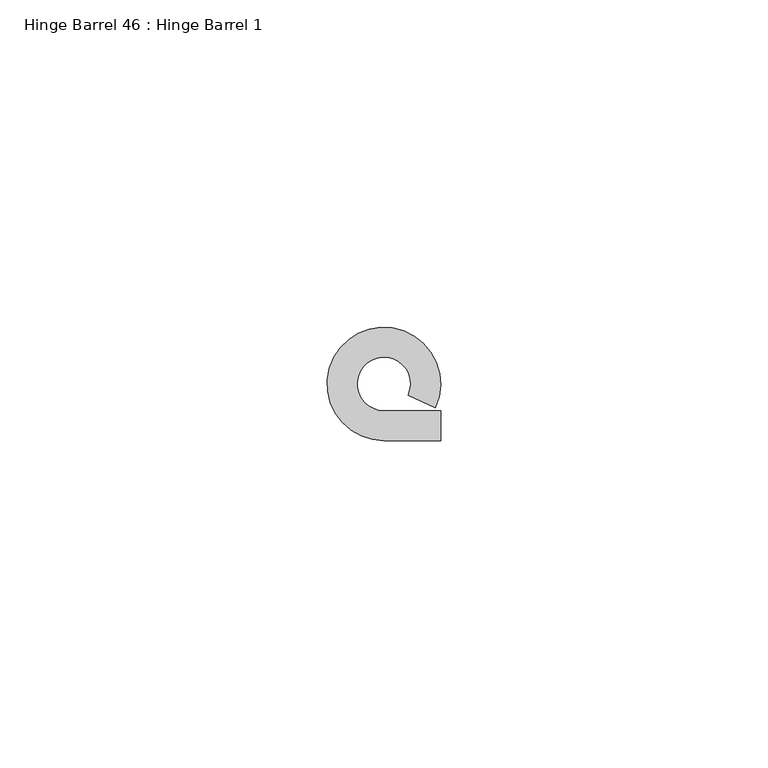
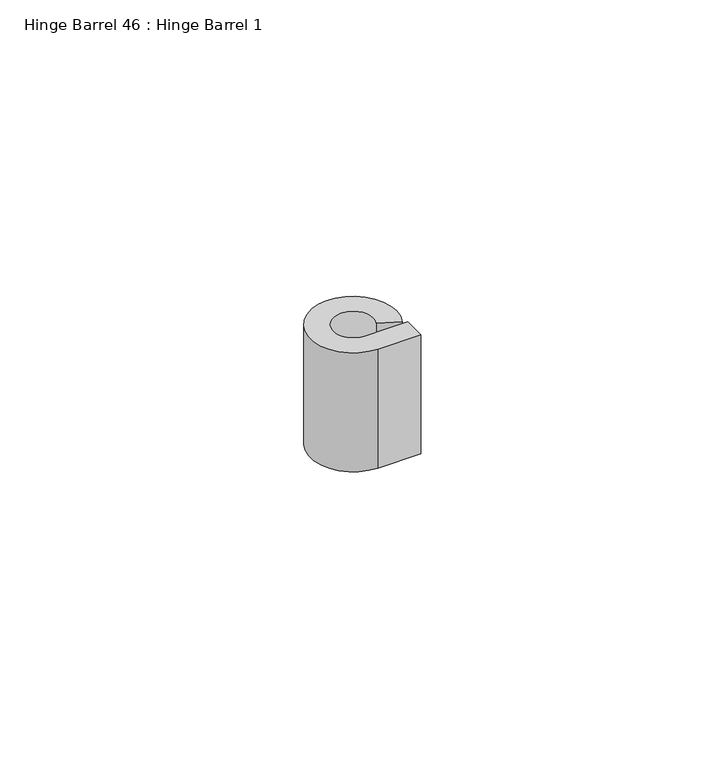
"""IFC4 building model written with IfcOpenShell, lengths in millimetres: proxy geometry, Hinge Barrel 46 : Hinge Barrel 1."""

from ifc_helpers import new_model, si_unit, point, frame, frame_2d, origin, place, context, project, spatial, polyline, circle_curve, trimmed, segment, composite_curve, outline, extrude, source, transform, mapped, element, save


def hinge_barrel_46_hinge_barrel_1_0a67a66c(model_context):
    return source(origin(), model_context, "Body", "SweptSolid", [
        extrude(outline(composite_curve([segment(polyline([(587323.2214739, -534104.7943841), (587327.7934739, -534104.7943841), (587327.7934739, -534109.3584466), (587319.1320739, -534109.3584466)]), True, "CONTINUOUS"), segment(trimmed(circle_curve(frame_2d((587319.1320739, -534100.7049841)), 8.6534625), [point((587319.1320739, -534109.3584466))], [point((587326.986084, -534104.3377433))], False, "CARTESIAN"), True, "CONTINUOUS"), segment(polyline([(587326.986084, -534104.3377433), (587322.8436736, -534102.421731)]), True, "CONTINUOUS"), segment(trimmed(circle_curve(frame_2d((587319.1320739, -534100.7049841)), 4.0894), [point((587322.8436736, -534102.421731))], [point((587319.1320739, -534104.7943841))], True, "CARTESIAN"), True, "CONTINUOUS"), segment(polyline([(587319.1320739, -534104.7943841), (587323.2214739, -534104.7943841)]), True, "CONTINUOUS")], self_intersect=False)), frame((0.0, 0.0, 2038.35), z_axis=(0.0, 0.0, 1.0), x_axis=(1.0, 0.0, 0.0)), (0.0, 0.0, 1.0), 25.4),
    ])


if __name__ == "__main__":
    model = new_model("IFC4")
    model_context = context("Model", 3, world=origin())
    ifc_project = project(units=[si_unit("LENGTHUNIT", "METRE", prefix="MILLI")], contexts=[model_context])
    site = spatial("IfcSite", under=ifc_project)
    building = spatial("IfcBuilding", under=site)
    placement = place(None, origin())
    hinge_barrel_46_hinge_barrel_1_shape = hinge_barrel_46_hinge_barrel_1_0a67a66c(model_context)
    element("IfcBuildingElementProxy", 1, Name="Hinge Barrel 46 : Hinge Barrel 1", ObjectType="Hinge Barrel 46 : Hinge Barrel 1", at=placement, inside=building, context=model_context, shape_type="MappedRepresentation", body=[
        mapped(hinge_barrel_46_hinge_barrel_1_shape, transform((0.0, 0.0, 0.0), x_axis=(1.0, 0.0, 0.0), y_axis=(0.0, 1.0, 0.0), z_axis=(0.0, 0.0, 1.0))),
    ])
    save(model, "model.ifc")

# Revit data of these elements
# Element 1 (IfcBuildingElementProxy, "Hinge Barrel 46 : Hinge Barrel 1")
#   Materials on its faces: "6\"X6\" WELD-ON STL BUTT HINGE"
# Materials
#   "6\"X6\" WELD-ON STL BUTT HINGE": class "Metal", colour RGB 189 187 185, transparency 0, Description = "Carbon steel", Cost = 0
